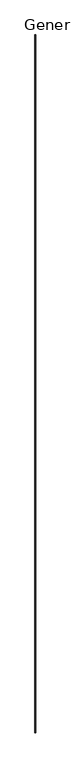
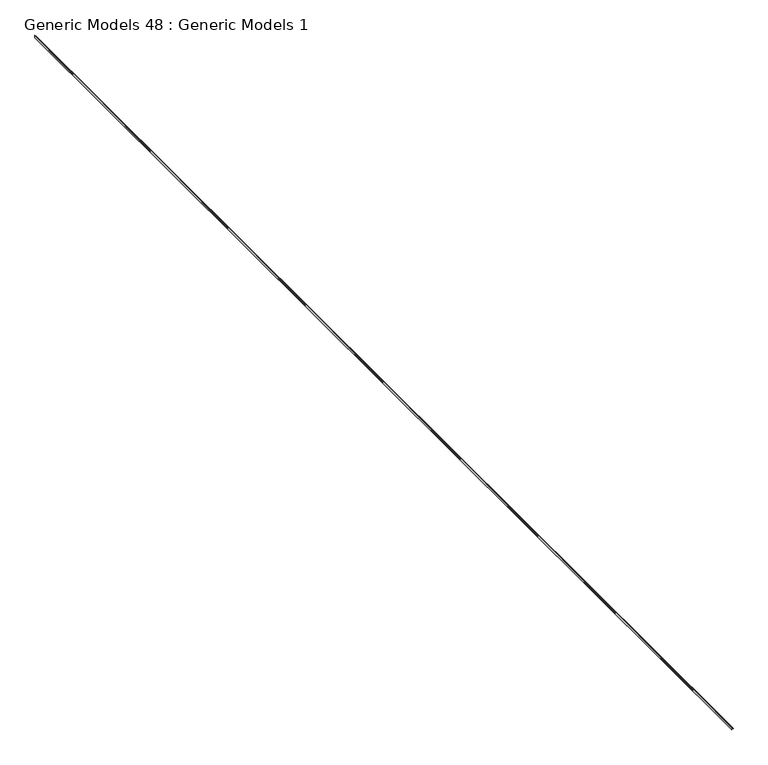
"""IFC4 building model written with IfcOpenShell, lengths in millimetres: proxy geometry, Generic Models 48 : Generic Models 1."""

from ifc_helpers import new_model, si_unit, origin, place, context, project, spatial, faceted_brep, source, transform, mapped, element, save


def generic_models_48_generic_models_1_d970f533(model_context):
    return source(origin(), model_context, "Body", "Brep", [
        faceted_brep([(-9255.2986296, 11981.8769662, 126375.541), (-9254.0286296, 11981.8769662, 126375.541), (-9254.0286296, 11981.8769662, 126356.491), (-9233.0736296, 11981.8769662, 126356.491), (-9233.0736296, 11981.8769662, 126351.7412), (-9234.3436296, 11981.8769662, 126351.7412), (-9234.3436296, 11981.8769662, 126355.221), (-9254.0286296, 11981.8769662, 126355.221), (-9254.0286296, 11981.8769662, 126336.171), (-9255.2986296, 11981.8769662, 126336.171), (-9255.2986296, -7068.1230338, 126375.541), (-9255.2986296, -7068.1230338, 126336.171), (-9254.0286296, -7068.1230338, 126336.171), (-9254.0286296, -7068.1230338, 126355.221), (-9234.3436296, -7068.1230338, 126355.221), (-9234.3436296, -7068.1230338, 126351.7412), (-9233.0736296, -7068.1230338, 126351.7412), (-9233.0736296, -7068.1230338, 126356.491), (-9254.0286296, -7068.1230338, 126356.491), (-9254.0286296, -7068.1230338, 126375.541), (-9233.0736296, -6864.9230338, 126351.7412), (-9233.0736296, 11778.6769662, 126351.7412), (-9234.3436296, -6864.9230338, 126351.7412), (-9234.3436296, 11778.6769662, 126351.7412), (-9234.3436296, -6864.9230338, 126355.221), (-9234.3436296, 11778.6769662, 126355.221)], [[[0, 1, 2, 3, 4, 5, 6, 7, 8, 9]], [[10, 11, 12, 13, 14, 15, 16, 17, 18, 19]], [[1, 0, 10, 19]], [[2, 1, 19, 18]], [[3, 2, 18, 17]], [[4, 3, 17, 16, 20, 21]], [[5, 4, 21, 20, 16, 15, 22, 23]], [[6, 5, 23, 22, 15, 14, 24, 25]], [[7, 6, 25, 24, 14, 13]], [[8, 7, 13, 12]], [[9, 8, 12, 11]], [[0, 9, 11, 10]]]),
    ])


if __name__ == "__main__":
    model = new_model("IFC4")
    model_context = context("Model", 3, world=origin())
    ifc_project = project(units=[si_unit("LENGTHUNIT", "METRE", prefix="MILLI")], contexts=[model_context])
    site = spatial("IfcSite", under=ifc_project)
    building = spatial("IfcBuilding", under=site)
    placement = place(None, origin())
    generic_models_48_generic_models_1_shape = generic_models_48_generic_models_1_d970f533(model_context)
    element("IfcBuildingElementProxy", 1, Name="Generic Models 48 : Generic Models 1", ObjectType="Generic Models 48 : Generic Models 1", at=placement, inside=building, context=model_context, shape_type="MappedRepresentation", body=[
        mapped(generic_models_48_generic_models_1_shape, transform((0.0, 0.0, 0.0), x_axis=(1.0, 0.0, 0.0), y_axis=(0.0, 1.0, 0.0), z_axis=(0.0, 0.0, 1.0))),
    ])
    save(model, "model.ifc")

# Revit data of these elements
# Element 1 (IfcBuildingElementProxy, "Generic Models 48 : Generic Models 1")
#   Materials on its faces: "_ 16 GA. COPPER VENTED T REVEAL BEAD (CONT. AROUND PERIMETER OF BEAM)"
# Materials
#   "_ 16 GA. COPPER VENTED T REVEAL BEAD (CONT. AROUND PERIMETER OF BEAM)": class "Generic", colour RGB 253 192 103, transparency 0, Cost = 0
